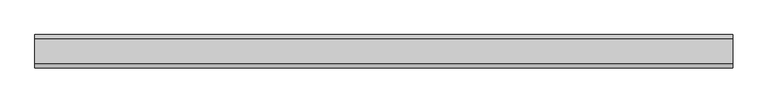
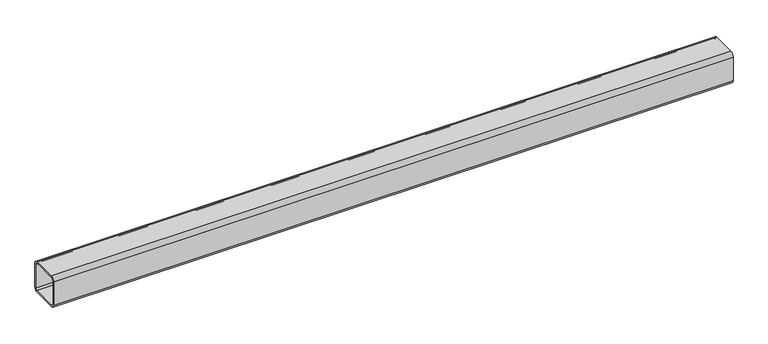
"""IFC4 building model written with IfcOpenShell, lengths in millimetres: beam geometry, Гнутый прямоугольный профиль (Трубы 30245-94) Балки : гнутый прямоуг. проф. 100x6."""

from ifc_helpers import new_model, si_unit, point, frame, frame_2d, origin, place, context, project, spatial, polyline, circle_curve, trimmed, segment, composite_curve, outline, extrude, source, transform, mapped, element, save


def beam_8faf6b92(model_context):
    return source(origin(), model_context, "Body", "SweptSolid", [
        extrude(outline(composite_curve([segment(polyline([(-38.0, 50.0), (38.0, 50.0)]), True, "CONTINUOUS"), segment(trimmed(circle_curve(frame_2d((38.0, 38.0)), 12.0), [point((38.0, 50.0))], [point((50.0, 38.0))], False, "CARTESIAN"), True, "CONTINUOUS"), segment(polyline([(50.0, 38.0), (50.0, -38.0)]), True, "CONTINUOUS"), segment(trimmed(circle_curve(frame_2d((38.0, -38.0)), 12.0), [point((50.0, -38.0))], [point((38.0, -50.0))], False, "CARTESIAN"), True, "CONTINUOUS"), segment(polyline([(38.0, -50.0), (-38.0, -50.0)]), True, "CONTINUOUS"), segment(trimmed(circle_curve(frame_2d((-38.0, -38.0)), 12.0), [point((-38.0, -50.0))], [point((-50.0, -38.0))], False, "CARTESIAN"), True, "CONTINUOUS"), segment(polyline([(-50.0, -38.0), (-50.0, 38.0)]), True, "CONTINUOUS"), segment(trimmed(circle_curve(frame_2d((-38.0, 38.0)), 12.0), [point((-50.0, 38.0))], [point((-38.0, 50.0))], False, "CARTESIAN"), True, "CONTINUOUS")], self_intersect=False), holes=[composite_curve([segment(trimmed(circle_curve(frame_2d((-38.0, 38.0)), 6.0), [point((-38.0, 44.0))], [point((-44.0, 38.0))], True, "CARTESIAN"), True, "CONTINUOUS"), segment(polyline([(-44.0, 38.0), (-44.0, -38.0)]), True, "CONTINUOUS"), segment(trimmed(circle_curve(frame_2d((-38.0, -38.0)), 6.0), [point((-44.0, -38.0))], [point((-38.0, -44.0))], True, "CARTESIAN"), True, "CONTINUOUS"), segment(polyline([(-38.0, -44.0), (38.0, -44.0)]), True, "CONTINUOUS"), segment(trimmed(circle_curve(frame_2d((38.0, -38.0)), 6.0), [point((38.0, -44.0))], [point((44.0, -38.0))], True, "CARTESIAN"), True, "CONTINUOUS"), segment(polyline([(44.0, -38.0), (44.0, 38.0)]), True, "CONTINUOUS"), segment(trimmed(circle_curve(frame_2d((38.0, 38.0)), 6.0), [point((44.0, 38.0))], [point((38.0, 44.0))], True, "CARTESIAN"), True, "CONTINUOUS"), segment(polyline([(38.0, 44.0), (-38.0, 44.0)]), True, "CONTINUOUS")], self_intersect=False)]), frame((-1047.5, 0.0, 0.0), z_axis=(1.0, 0.0, 0.0), x_axis=(0.0, 1.0, 0.0)), (0.0, 0.0, 1.0), 2095.0),
    ])


if __name__ == "__main__":
    model = new_model("IFC4")
    model_context = context("Model", 3, world=origin())
    ifc_project = project(units=[si_unit("LENGTHUNIT", "METRE", prefix="MILLI")], contexts=[model_context])
    site = spatial("IfcSite", under=ifc_project)
    building = spatial("IfcBuilding", under=site)
    placement = place(None, origin())
    beam_shape = beam_8faf6b92(model_context)
    element("IfcBeam", 1, ObjectType="Гнутый прямоугольный профиль (Трубы 30245-94) Балки : гнутый прямоуг. проф. 100x6", at=placement, inside=building, context=model_context, shape_type="MappedRepresentation", body=[
        mapped(beam_shape, transform((0.0, 0.0, 0.0), x_axis=(1.0, 0.0, 0.0), y_axis=(0.0, 1.0, 0.0), z_axis=(0.0, 0.0, 1.0))),
    ])
    save(model, "model.ifc")

# Revit data of these elements
# Type "Гнутый прямоугольный профиль (Трубы 30245-94) Балки : гнутый прямоуг. проф. 100x6"
#   ri = 12 mm
#   ra = 6 mm
#   W = 0.173578
#   Vz = 50 mm
#   Vy = 50 mm
#   Vpz = 50 mm
#   Vpy = 50 mm
#   Length [instance default] = 1500 mm
#   bf = 100 mm
#   d = 100 mm
#   tf = 6 mm
#   tw = 6 mm
#   A = 0.00226 m²
#   Structural Material [instance default] = Металл - Сталь - 345 МПa
#   Assembly Code = ""
# Element 1 (IfcBeam, "Гнутый прямоугольный профиль (Трубы 30245-94) Балки : гнутый прямоуг. проф. 100x6")
#   Structural Material = C235
#   Materials on its faces: "C235"
# Materials
#   "Металл - Сталь - 345 МПa": class "Металл", colour RGB 247 247 247, transparency 0
#   "C235": class "Не назначено", colour RGB 0 0 0, transparency 0
